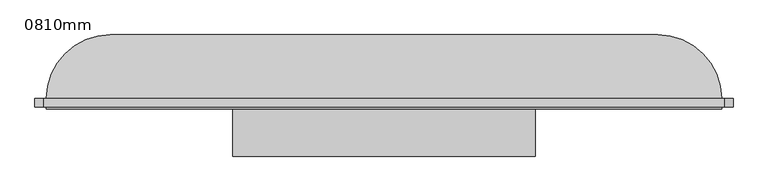
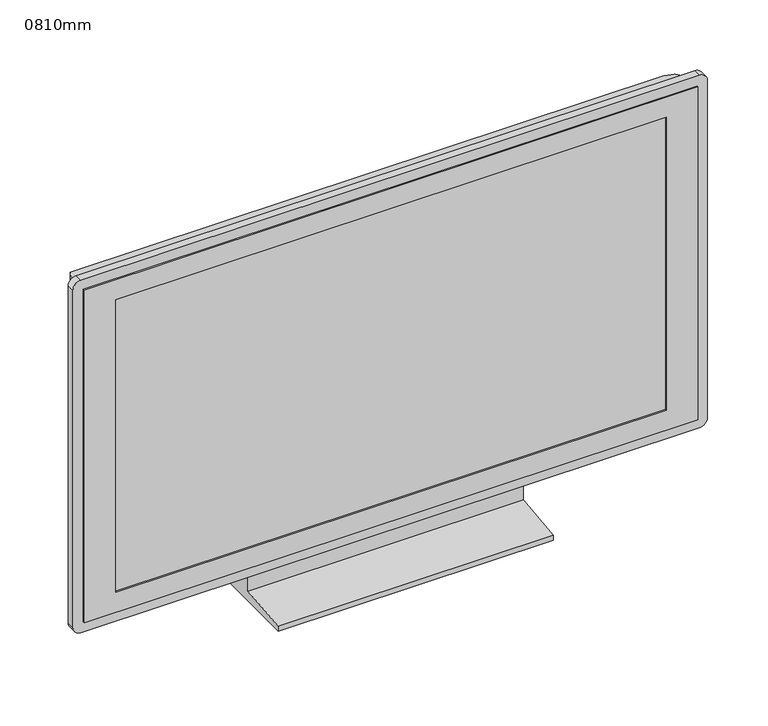
"""IFC4 building model written with IfcOpenShell, lengths in millimetres: furniture geometry, M_TV - Flat Screen : 0810mm."""

from ifc_helpers import new_model, si_unit, point, frame, frame_2d, origin, place, context, project, spatial, polyline, circle_curve, ellipse_curve, trimmed, segment, composite_curve, outline, extrude, faceted_brep, source, transform, mapped, element, save
from ifc_brep_helpers import plane_surface, cylinder_surface, advanced_brep


def furniture_0810mm_d9060323(model_context):
    return source(origin(), model_context, "Body", "SolidModel", [
        advanced_brep(
        [(-586.8783027, -51.4613764, 80.0), (578.9892744, -51.4613764, 80.0), (578.9892744, -51.4613764, 748.3544945), (-586.8783027, -51.4613764, 748.3544945), (468.9892744, 58.5386236, 80.0), (-476.8783027, 58.5386236, 80.0), (-476.8783027, 58.5386236, 638.3544945), (468.9892744, 58.5386236, 638.3544945)],
        [
            (0, 1),
            (1, 2),
            (2, 3),
            (3, 0),
            (4, 5),
            (5, 6),
            (6, 7),
            (7, 4),
            (0, 5, circle_curve(frame((-476.8783027, -51.4613764, 80.0), z_axis=(0.0, 0.0, -1.0), x_axis=(-1.0, 0.0, 0.0)), 110.0)),
            (4, 1, circle_curve(frame((468.9892744, -51.4613764, 80.0), z_axis=(0.0, 0.0, -1.0), x_axis=(1.0, 0.0, 0.0)), 110.0)),
            (7, 2, ellipse_curve(frame((468.9892744, -51.4613764, 638.3544945), z_axis=(0.7071067811865475, 0.0, -0.7071067811865475), x_axis=(0.7071067811865474, 0.0, 0.7071067811865476)), 155.5634919, 110.0)),
            (6, 3, ellipse_curve(frame((-476.8783027, -51.4613764, 638.3544945), z_axis=(0.7071067811865475, 0.0, 0.7071067811865476), x_axis=(-0.7071067811865476, 0.0, 0.7071067811865475)), 155.5634919, 110.0)),
        ],
        [
            plane_surface(frame((-586.8783027, -51.4613764, 748.3544945), z_axis=(0.0, -1.0, 0.0), x_axis=(-1.0, 0.0, 0.0))),
            plane_surface(frame((-586.8783027, 58.5386236, 748.3544945), z_axis=(0.0, 1.0, 0.0), x_axis=(1.0, 0.0, 0.0))),
            plane_surface(frame((-586.8783027, -51.4613764, 80.0), z_axis=(0.0, 0.0, -1.0), x_axis=(0.0, 1.0, 0.0))),
            cylinder_surface(frame((468.9892744, -51.4613764, 80.0), z_axis=(0.0, 0.0, 1.0), x_axis=(1.0, 0.0, 0.0)), 110.0),
            cylinder_surface(frame((578.9892744, -51.4613764, 638.3544945), z_axis=(-1.0, 0.0, 0.0), x_axis=(0.0, 0.0, 1.0)), 110.0),
            cylinder_surface(frame((-476.8783027, -51.4613764, 748.3544945), z_axis=(0.0, 0.0, -1.0), x_axis=(-1.0, 0.0, 0.0)), 110.0),
        ],
        [
            (0, [[1, 2, 3, 4]]),
            (1, [[5, 6, 7, 8]]),
            (2, [[-1, 9, -5, 10]]),
            (3, [[11, -2, -10, -8]]),
            (4, [[-11, -7, 12, -3]]),
            (5, [[-12, -6, -9, -4]]),
        ],
    ),
        extrude(outline(composite_curve([segment(polyline([(768.3544945, 583.9892744), (768.3544945, -591.8783027)]), True, "CONTINUOUS"), segment(trimmed(circle_curve(frame_2d((753.3544945, -591.8783027)), 15.0), [point((768.3544945, -591.8783027))], [point((753.3544945, -606.8783027))], False, "CARTESIAN"), True, "CONTINUOUS"), segment(polyline([(753.3544945, -606.8783027), (75.0, -606.8783027)]), True, "CONTINUOUS"), segment(trimmed(circle_curve(frame_2d((75.0, -591.8783027)), 15.0), [point((75.0, -606.8783027))], [point((60.0, -591.8783027))], False, "CARTESIAN"), True, "CONTINUOUS"), segment(polyline([(60.0, -591.8783027), (60.0, 583.9892744)]), True, "CONTINUOUS"), segment(trimmed(circle_curve(frame_2d((75.0, 583.9892744)), 15.0), [point((60.0, 583.9892744))], [point((75.0, 598.9892744))], False, "CARTESIAN"), True, "CONTINUOUS"), segment(polyline([(75.0, 598.9892744), (753.3544945, 598.9892744)]), True, "CONTINUOUS"), segment(trimmed(circle_curve(frame_2d((753.3544945, 583.9892744)), 15.0), [point((753.3544945, 598.9892744))], [point((768.3544945, 583.9892744))], False, "CARTESIAN"), True, "CONTINUOUS")], self_intersect=False), holes=[polyline([(748.3544945, 578.9892744), (80.0, 578.9892744), (80.0, -586.8783027), (748.3544945, -586.8783027), (748.3544945, 578.9892744)])]), frame((0.0, -66.4613764, 0.0), z_axis=(0.0, 1.0, 0.0), x_axis=(0.0, 0.0, 1.0)), (0.0, 0.0, 1.0), 15.0),
        faceted_brep([(578.9892744, -69.4613764, 748.3544945), (-586.8783027, -69.4613764, 748.3544945), (-586.8783027, -69.4613764, 80.0), (578.9892744, -69.4613764, 80.0), (-526.8783027, -69.4613764, 708.3544945), (518.9892744, -69.4613764, 708.3544945), (518.9892744, -69.4613764, 120.0), (-526.8783027, -69.4613764, 120.0), (578.9892744, -51.4613764, 748.3544945), (578.9892744, -51.4613764, 80.0), (-586.8783027, -51.4613764, 80.0), (-586.8783027, -51.4613764, 748.3544945), (-526.8783027, -66.4613764, 708.3544945), (-526.8783027, -66.4613764, 120.0), (518.9892744, -66.4613764, 120.0), (518.9892744, -66.4613764, 708.3544945)], [[[0, 1, 2, 3], [4, 5, 6, 7]], [[8, 9, 10, 11]], [[1, 0, 8, 11]], [[2, 1, 11, 10]], [[3, 2, 10, 9]], [[0, 3, 9, 8]], [[12, 13, 14, 15]], [[12, 15, 5, 4]], [[15, 14, 6, 5]], [[14, 13, 7, 6]], [[13, 12, 4, 7]]]),
        extrude(outline(polyline([(-51.4613764, 80.0), (-1.4613764, 80.0), (48.5386236, 0.0), (-151.4613764, 0.0), (-151.4613764, 10.0), (-51.4613764, 20.0), (-51.4613764, 80.0)])), frame((-265.4114084, 0.0, 0.0), z_axis=(1.0, 0.0, 0.0), x_axis=(0.0, 1.0, 0.0)), (0.0, 0.0, 1.0), 522.9337886),
    ])


if __name__ == "__main__":
    model = new_model("IFC4")
    model_context = context("Model", 3, world=origin())
    ifc_project = project(units=[si_unit("LENGTHUNIT", "METRE", prefix="MILLI")], contexts=[model_context])
    site = spatial("IfcSite", under=ifc_project)
    building = spatial("IfcBuilding", under=site)
    placement = place(None, origin())
    furniture_0810mm_shape = furniture_0810mm_d9060323(model_context)
    element("IfcFurniture", 1, ObjectType="M_TV - Flat Screen : 0810mm", at=placement, inside=building, context=model_context, shape_type="MappedRepresentation", body=[
        mapped(furniture_0810mm_shape, transform((0.0, 0.0, 0.0), x_axis=(1.0, 0.0, 0.0), y_axis=(0.0, 1.0, 0.0), z_axis=(0.0, 0.0, 1.0))),
    ])
    save(model, "model.ifc")

# Revit data of these elements
# Type "M_TV - Flat Screen : 0810mm"
#   SinAng = 0.049 cm
#   L = 104.5868 cm
#   H = 58.8354 cm
#   Thickness = 11 cm
#   Diagonal = 120 cm
#   Default Elevation = 60 cm
#   CosAng = 0.0872 cm
#   Stand [instance default] = yes
# Element 1 (IfcFurniture, "M_TV - Flat Screen : 0810mm")
#   Materials on its faces: "TV - Black", "TV - Glass", "TV - Screen"
# Materials
#   "TV - Black": class "Miscellaneous", colour RGB 49 49 49, transparency 0
#   "TV - Glass": class "Miscellaneous", colour RGB 157 157 157, transparency 0.9
#   "TV - Screen": class "Miscellaneous", colour RGB 0 0 0, transparency 0
